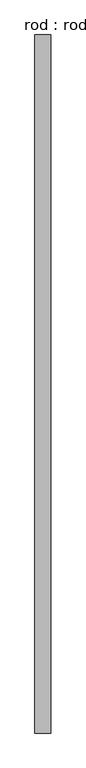
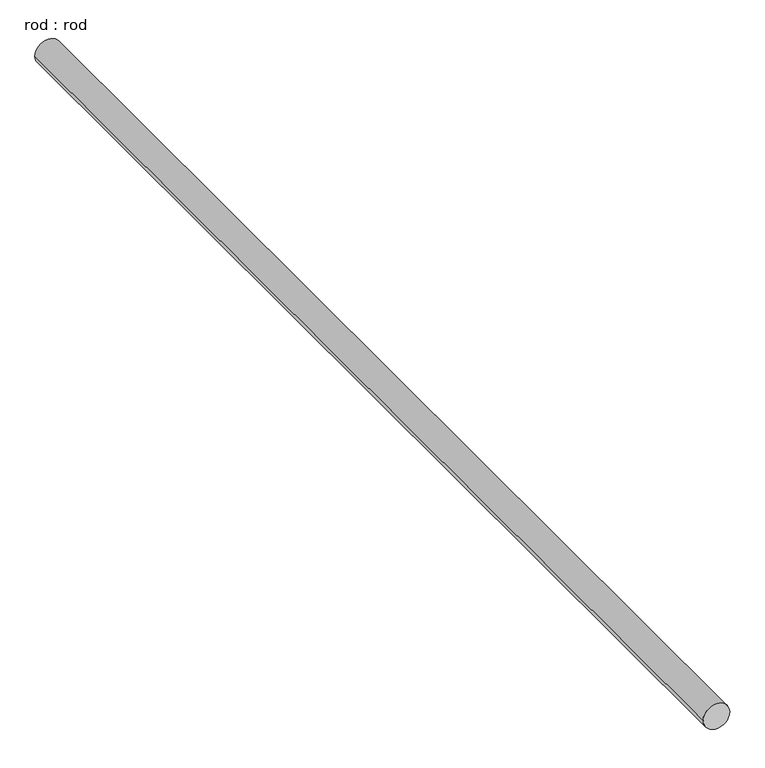
"""IFC4 building model written with IfcOpenShell, lengths in millimetres: proxy geometry, rod : rod."""

from ifc_helpers import new_model, si_unit, point, frame, frame_2d, origin, place, context, project, spatial, circle_curve, trimmed, segment, composite_curve, outline, extrude, source, transform, mapped, element, save


def rod_rod_7f2afdde(model_context):
    return source(origin(), model_context, "Body", "SweptSolid", [
        extrude(outline(composite_curve([segment(trimmed(circle_curve(frame_2d((0.0108462, 0.0)), 200.0), [point((0.0108462, 200.0))], [point((0.0108462, -200.0))], False, "CARTESIAN"), True, "CONTINUOUS"), segment(trimmed(circle_curve(frame_2d((0.0108462, 0.0)), 200.0), [point((0.0108462, -200.0))], [point((0.0108462, 200.0))], False, "CARTESIAN"), True, "CONTINUOUS")], self_intersect=False)), frame((0.0, -4666.1999561, 0.0), z_axis=(0.0, 1.0, 0.0), x_axis=(0.0, 0.0, 1.0)), (0.0, 0.0, 1.0), 17517.8571429),
    ])


if __name__ == "__main__":
    model = new_model("IFC4")
    model_context = context("Model", 3, world=origin())
    ifc_project = project(units=[si_unit("LENGTHUNIT", "METRE", prefix="MILLI")], contexts=[model_context])
    site = spatial("IfcSite", under=ifc_project)
    building = spatial("IfcBuilding", under=site)
    placement = place(None, origin())
    rod_rod_shape = rod_rod_7f2afdde(model_context)
    element("IfcBuildingElementProxy", 1, Name="rod : rod", ObjectType="rod : rod", at=placement, inside=building, context=model_context, shape_type="MappedRepresentation", body=[
        mapped(rod_rod_shape, transform((0.0, 0.0, 0.0), x_axis=(1.0, 0.0, 0.0), y_axis=(0.0, 1.0, 0.0), z_axis=(0.0, 0.0, 1.0))),
    ])
    save(model, "model.ifc")

# Revit data of these elements
# Type "rod : rod"
#   Default Elevation = 0
